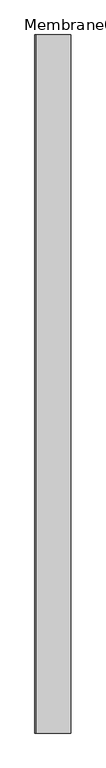
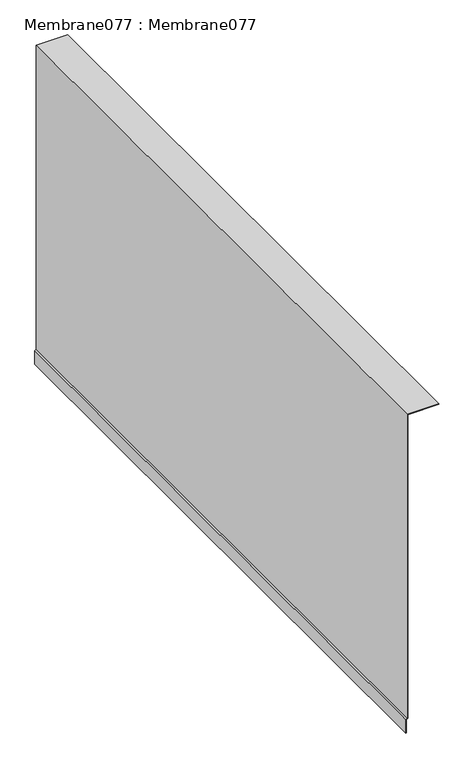
"""IFC4 building model written with IfcOpenShell, lengths in millimetres: proxy geometry, Membrane077 : Membrane077."""

from ifc_helpers import new_model, si_unit, frame, origin, place, context, project, spatial, polyline, outline, extrude, source, transform, mapped, element, save


def membrane077_membrane077_444aef54(model_context):
    return source(origin(), model_context, "Body", "SweptSolid", [
        extrude(outline(polyline([(40165.0, 10140.0400391), (40165.0, 10041.5058594), (39165.9001666, 10041.5058594), (39161.9011432, 10037.5068359), (39118.5507813, 10037.5068359), (39118.5507813, 10039.0068359), (39161.2783203, 10039.0068359), (39165.2773438, 10043.0058594), (40163.5, 10043.0058594), (40163.5, 10140.0400391), (40165.0, 10140.0400391)])), frame((0.0, 2217.3609988, 0.0), z_axis=(0.0, 1.0, 0.0), x_axis=(0.0, 0.0, 1.0)), (0.0, 0.0, 1.0), 2000.0),
    ])


if __name__ == "__main__":
    model = new_model("IFC4")
    model_context = context("Model", 3, world=origin())
    ifc_project = project(units=[si_unit("LENGTHUNIT", "METRE", prefix="MILLI")], contexts=[model_context])
    site = spatial("IfcSite", under=ifc_project)
    building = spatial("IfcBuilding", under=site)
    placement = place(None, origin())
    membrane077_membrane077_shape = membrane077_membrane077_444aef54(model_context)
    element("IfcBuildingElementProxy", 1, Name="Membrane077 : Membrane077", ObjectType="Membrane077 : Membrane077", at=placement, inside=building, context=model_context, shape_type="MappedRepresentation", body=[
        mapped(membrane077_membrane077_shape, transform((0.0, 0.0, 0.0), x_axis=(1.0, 0.0, 0.0), y_axis=(0.0, 1.0, 0.0), z_axis=(0.0, 0.0, 1.0))),
    ])
    save(model, "model.ifc")

# Revit data of these elements
# Type "Membrane077 : Membrane077"
#   NameOverride = "Membrane077"
# Element 1 (IfcBuildingElementProxy, "Membrane077 : Membrane077")
#   Materials on its faces: "(2) LAYERS OF ICE & WATER SHIELD (BITUTHANE) UNDER STUCCO"
# Materials
#   "(2) LAYERS OF ICE & WATER SHIELD (BITUTHANE) UNDER STUCCO": class "Unassigned", colour RGB 186 255 159, transparency 0, Cost = 0
